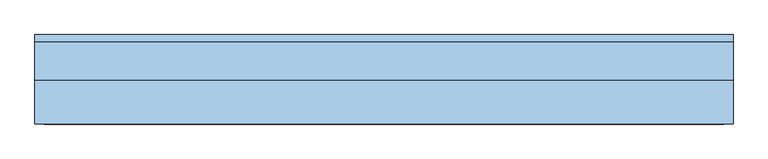
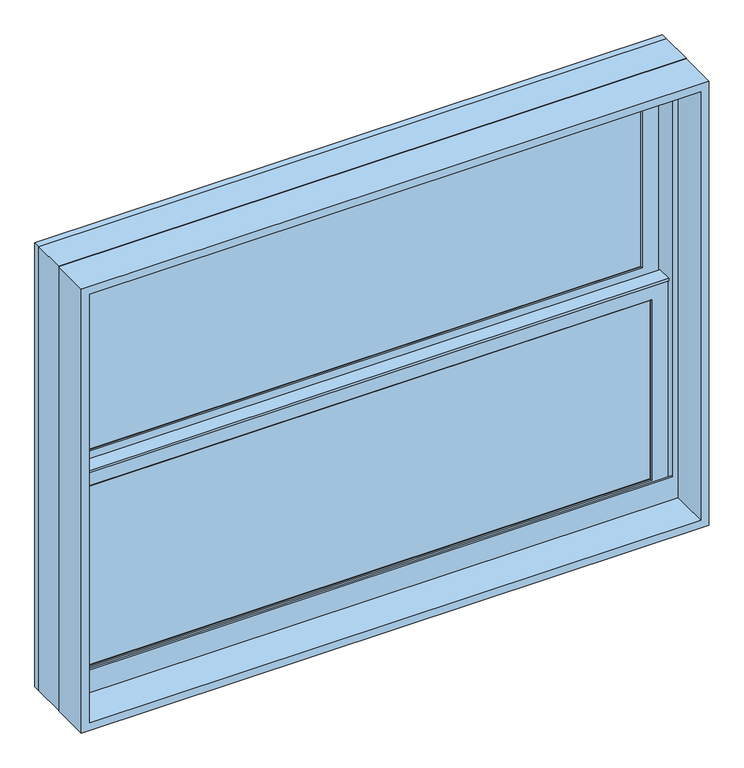
"""IFC4 building model written with IfcOpenShell, lengths in millimetres: window geometry, Window-Double_Hung-Marvin-Essential : ESDH4030."""

from ifc_helpers import new_model, si_unit, frame, origin, place, context, project, spatial, polyline, outline, extrude, faceted_brep, source, transform, mapped, element, save


def window_916ece20(model_context):
    return source(origin(), model_context, "Body", "SolidModel", [
        extrude(outline(polyline([(191.5583333, 20.6375), (191.5583333, 15.875), (172.5083333, 15.875), (172.5083333, 20.6375), (191.5583333, 20.6375)])), frame((0.0, 0.0, 1593.85), z_axis=(0.0, 0.0, 1.0), x_axis=(1.0, 0.0, 0.0)), (0.0, 0.0, 1.0), 374.65),
        extrude(outline(polyline([(-172.5083333, 20.6375), (-172.5083333, 15.875), (-191.5583333, 15.875), (-191.5583333, 20.6375), (-172.5083333, 20.6375)])), frame((0.0, 0.0, 1593.85), z_axis=(0.0, 0.0, 1.0), x_axis=(1.0, 0.0, 0.0)), (0.0, 0.0, 1.0), 374.65),
        extrude(outline(polyline([(546.1, 20.6375), (546.1, 15.875), (-546.1, 15.875), (-546.1, 20.6375), (546.1, 20.6375)])), frame((0.0, 0.0, 1771.65), z_axis=(0.0, 0.0, 1.0), x_axis=(1.0, 0.0, 0.0)), (0.0, 0.0, 1.0), 19.05),
        extrude(outline(polyline([(-191.5583333, 46.83125), (-191.5583333, 51.59375), (-172.5083333, 51.59375), (-172.5083333, 46.83125), (-191.5583333, 46.83125)])), frame((0.0, 0.0, 2006.6), z_axis=(0.0, 0.0, 1.0), x_axis=(1.0, 0.0, 0.0)), (0.0, 0.0, 1.0), 374.65),
        extrude(outline(polyline([(172.5083333, 46.83125), (172.5083333, 51.59375), (191.5583333, 51.59375), (191.5583333, 46.83125), (172.5083333, 46.83125)])), frame((0.0, 0.0, 2006.6), z_axis=(0.0, 0.0, 1.0), x_axis=(1.0, 0.0, 0.0)), (0.0, 0.0, 1.0), 374.65),
        extrude(outline(polyline([(-546.1, 46.83125), (-546.1, 51.59375), (546.1, 51.59375), (546.1, 46.83125), (-546.1, 46.83125)])), frame((0.0, 0.0, 2184.4), z_axis=(0.0, 0.0, 1.0), x_axis=(1.0, 0.0, 0.0)), (0.0, 0.0, 1.0), 19.05),
        extrude(outline(polyline([(191.5583333, 20.6375), (172.5083333, 20.6375), (172.5083333, 25.4), (191.5583333, 25.4), (191.5583333, 20.6375)])), frame((0.0, 0.0, 1593.85), z_axis=(0.0, 0.0, 1.0), x_axis=(1.0, 0.0, 0.0)), (0.0, 0.0, 1.0), 374.65),
        extrude(outline(polyline([(-172.5083333, 20.6375), (-191.5583333, 20.6375), (-191.5583333, 25.4), (-172.5083333, 25.4), (-172.5083333, 20.6375)])), frame((0.0, 0.0, 1593.85), z_axis=(0.0, 0.0, 1.0), x_axis=(1.0, 0.0, 0.0)), (0.0, 0.0, 1.0), 374.65),
        extrude(outline(polyline([(546.1, 20.6375), (-546.1, 20.6375), (-546.1, 25.4), (546.1, 25.4), (546.1, 20.6375)])), frame((0.0, 0.0, 1771.65), z_axis=(0.0, 0.0, 1.0), x_axis=(1.0, 0.0, 0.0)), (0.0, 0.0, 1.0), 19.05),
        extrude(outline(polyline([(-191.5583333, 56.35625), (-172.5083333, 56.35625), (-172.5083333, 51.59375), (-191.5583333, 51.59375), (-191.5583333, 56.35625)])), frame((0.0, 0.0, 2006.6), z_axis=(0.0, 0.0, 1.0), x_axis=(1.0, 0.0, 0.0)), (0.0, 0.0, 1.0), 374.65),
        extrude(outline(polyline([(172.5083333, 56.35625), (191.5583333, 56.35625), (191.5583333, 51.59375), (172.5083333, 51.59375), (172.5083333, 56.35625)])), frame((0.0, 0.0, 2006.6), z_axis=(0.0, 0.0, 1.0), x_axis=(1.0, 0.0, 0.0)), (0.0, 0.0, 1.0), 374.65),
        extrude(outline(polyline([(-546.1, 56.35625), (546.1, 56.35625), (546.1, 51.59375), (-546.1, 51.59375), (-546.1, 56.35625)])), frame((0.0, 0.0, 2184.4), z_axis=(0.0, 0.0, 1.0), x_axis=(1.0, 0.0, 0.0)), (0.0, 0.0, 1.0), 19.05),
        faceted_brep([(-573.0875, 5.6780605, 1998.5351748), (-573.0875, 5.6780605, 1993.9), (573.0875, 5.6780605, 1993.9), (573.0875, 5.6780605, 1998.5351748), (-573.0875, 34.8118605, 1998.5351748), (573.0875, 34.8118605, 1998.5351748), (573.0875, 34.8118605, 1993.9), (-573.0875, 34.8118605, 1993.9), (-573.0875, 30.1625, 1993.9), (-573.0875, 30.1625, 1566.8625), (-573.0875, 8.9241104, 1566.8625), (-573.0875, 8.9241104, 1993.9), (573.0875, 8.9241104, 1993.9), (573.0875, 30.1625, 1993.9), (573.0875, 8.9241104, 1566.8625), (573.0875, 30.1625, 1566.8625), (-557.2034752, 11.90625, 1979.6034752), (-557.2034752, 30.1625, 1979.6034752), (557.2034752, 30.1625, 1979.6034752), (557.2034752, 11.90625, 1979.6034752), (-540.54375, 10.4662439, 1962.94375), (-540.54375, 11.90625, 1962.94375), (540.54375, 11.90625, 1962.94375), (540.54375, 10.4662439, 1962.94375), (542.0858834, 8.9241104, 1964.4858834), (-542.0858834, 8.9241104, 1964.4858834), (557.2034752, 30.1625, 1582.7465248), (557.2034752, 11.90625, 1582.7465248), (540.54375, 11.90625, 1599.40625), (540.54375, 10.4662439, 1599.40625), (542.0858834, 8.9241104, 1597.8641166), (-557.2034752, 30.1625, 1582.7465248), (-557.2034752, 11.90625, 1582.7465248), (-540.54375, 11.90625, 1599.40625), (-540.54375, 10.4662439, 1599.40625), (-542.0858834, 8.9241104, 1597.8641166)], [[[0, 1, 2, 3]], [[4, 5, 6, 7]], [[1, 0, 4, 7, 8, 9, 10, 11]], [[2, 1, 11, 12]], [[7, 6, 13, 8]], [[3, 2, 12, 14, 15, 13, 6, 5]], [[0, 3, 5, 4]], [[16, 17, 18, 19]], [[20, 21, 22, 23]], [[20, 23, 24, 25]], [[19, 18, 26, 27]], [[23, 22, 28, 29]], [[24, 23, 29, 30]], [[27, 26, 31, 32]], [[29, 28, 33, 34]], [[30, 29, 34, 35]], [[15, 14, 10, 9]], [[15, 9, 8, 13], [18, 17, 31, 26]], [[17, 16, 32, 31]], [[16, 19, 27, 32], [22, 21, 33, 28]], [[21, 20, 34, 33]], [[20, 25, 35, 34]], [[10, 14, 12, 11], [25, 24, 30, 35]]]),
        extrude(outline(polyline([(38.5955581, 1979.6125), (33.5778968, 1979.6125), (33.5778968, 1981.2), (39.9405976, 1981.2), (39.9405976, 1979.6125), (61.515625, 1979.6125), (47.6307501, 1976.2975159), (38.5955581, 1976.2975159), (38.5955581, 1979.6125)])), frame((-573.0875, 0.0, 0.0), z_axis=(1.0, 0.0, 0.0), x_axis=(0.0, 1.0, 0.0)), (0.0, 0.0, 1.0), 1146.175),
        faceted_brep([(603.25, 0.0, 1536.7), (603.25, 0.0, 2438.4), (-603.25, 0.0, 2438.4), (-603.25, 0.0, 1536.7), (577.05625, 0.0, 1597.81875), (-577.05625, 0.0, 1597.81875), (-577.05625, 0.0, 2412.20625), (577.05625, 0.0, 2412.20625), (577.05625, 3.96875, 1536.7), (-577.05625, 3.96875, 1536.7), (-577.05625, 3.96875, 1597.81875), (577.05625, 3.96875, 1597.81875), (-603.25, 65.6828125, 1536.7), (-577.05625, 65.6828125, 1536.7), (577.05625, 65.6828125, 1536.7), (603.25, 65.6828125, 1536.7), (-603.25, 65.6828125, 2438.4), (603.25, 65.6828125, 2438.4), (577.05625, 65.6828125, 2412.20625), (-577.05625, 65.6828125, 2412.20625)], [[[0, 1, 2, 3], [4, 5, 6, 7]], [[8, 9, 10, 11]], [[5, 4, 11, 10]], [[0, 3, 12, 13, 9, 8, 14, 15]], [[13, 12, 16, 17, 15, 14, 18, 19]], [[13, 19, 6, 5, 10, 9]], [[7, 6, 19, 18]], [[18, 14, 8, 11, 4, 7]], [[1, 0, 15, 17]], [[2, 1, 17, 16]], [[3, 2, 16, 12]]]),
        faceted_brep([(577.05625, 30.1625, 1987.55), (575.46875, 30.1625, 1987.55), (575.46875, 30.1625, 1561.0544613), (577.05625, 30.1625, 1561.0544613), (-575.46875, 30.1625, 1987.55), (-577.05625, 30.1625, 1987.55), (-577.05625, 30.1625, 1561.0544613), (-575.46875, 30.1625, 1561.0544613), (575.46875, 63.5, 1987.55), (577.05625, 63.5, 1987.55), (577.05625, 63.5, 1554.5743077), (575.46875, 63.5, 1554.5743077), (-577.05625, 63.5, 1987.55), (-575.46875, 63.5, 1987.55), (-575.46875, 63.5, 1554.5743077), (-577.05625, 63.5, 1554.5743077), (588.3108932, 3.96875, 1566.1460105), (588.3108932, 3.96875, 1536.7), (588.3108932, 65.6828125, 1536.7), (588.3108932, 65.6828125, 1554.150012), (-588.3108932, 3.96875, 1536.7), (-588.3108932, 3.96875, 1566.1460105), (-588.3108932, 65.6828125, 1554.150012), (-588.3108932, 65.6828125, 1536.7), (588.3108932, 78.58125, 1551.6428097), (-588.3108932, 78.58125, 1551.6428097), (-586.2971252, 68.2348864, 1553.6539391), (-568.33135, 68.2348864, 1553.6539391), (-568.33135, 65.6828125, 1554.150012), (568.33135, 65.6828125, 1554.150012), (568.33135, 68.2348864, 1553.6539391), (586.2971252, 68.2348864, 1553.6539391), (-603.25, 65.6828125, 1536.7), (-603.25, 78.5948249, 1536.7), (603.25, 78.5948249, 1536.7), (603.25, 65.6828125, 1536.7), (-603.25, 78.58125, 2438.4), (603.25, 78.58125, 2438.4), (588.3108932, 78.58125, 2423.4608932), (-588.3108932, 78.58125, 2423.4608932), (-603.25, 65.6828125, 2438.4), (-586.2971252, 68.2348864, 2421.4471252), (586.2971252, 68.2348864, 2421.4471252), (568.33135, 68.2348864, 2403.48135), (-568.33135, 68.2348864, 2403.48135), (-568.33135, 65.6828125, 2403.48135), (568.33135, 65.6828125, 2403.48135), (603.25, 65.6828125, 2438.4)], [[[0, 1, 2, 3]], [[4, 5, 6, 7]], [[8, 9, 10, 11]], [[12, 13, 14, 15]], [[1, 8, 11, 2]], [[9, 0, 3, 10]], [[1, 0, 9, 8]], [[5, 4, 13, 12]], [[5, 12, 15, 6]], [[13, 4, 7, 14]], [[16, 17, 18, 19]], [[20, 21, 22, 23]], [[24, 25, 26, 27, 28, 22, 21, 16, 19, 29, 30, 31], [3, 2, 11, 10], [7, 6, 15, 14]], [[17, 16, 21, 20]], [[17, 20, 23, 32, 33, 34, 35, 18]], [[34, 33, 36, 37], [25, 24, 38, 39]], [[33, 32, 40, 36]], [[39, 41, 26, 25]], [[41, 42, 31, 30, 43, 44, 27, 26]], [[44, 45, 28, 27]], [[40, 32, 23, 22, 28, 45, 46, 29, 19, 18, 35, 47]], [[36, 40, 47, 37]], [[39, 38, 42, 41]], [[44, 43, 46, 45]], [[34, 37, 47, 35]], [[42, 38, 24, 31]], [[46, 43, 30, 29]]]),
        extrude(outline(polyline([(553.24375, 11.90625), (-553.24375, 11.90625), (-553.24375, 15.08125), (553.24375, 15.08125), (553.24375, 11.90625)])), frame((0.0, 0.0, 1586.70625), z_axis=(0.0, 0.0, 1.0), x_axis=(1.0, 0.0, 0.0)), (0.0, 0.0, 1.0), 388.9375),
        extrude(outline(polyline([(553.24375, 42.8625), (-553.24375, 42.8625), (-553.24375, 46.0375), (553.24375, 46.0375), (553.24375, 42.8625)])), frame((0.0, 0.0, 1999.45625), z_axis=(0.0, 0.0, 1.0), x_axis=(1.0, 0.0, 0.0)), (0.0, 0.0, 1.0), 388.9375),
        faceted_brep([(-540.54375, 31.194477, 1962.94375), (-542.0858834, 32.7366104, 1964.4858834), (542.0858834, 32.7366104, 1964.4858834), (540.54375, 31.194477, 1962.94375), (-540.54375, 30.1625, 1962.94375), (540.54375, 30.1625, 1962.94375), (-573.0875, 32.7366104, 1995.4875), (-573.0875, 30.1625, 1995.4875), (573.0875, 30.1625, 1995.4875), (573.0875, 32.7366104, 1995.4875), (542.0858834, 32.7366104, 1597.8641166), (540.54375, 31.194477, 1599.40625), (540.54375, 30.1625, 1599.40625), (573.0875, 30.1625, 1566.8625), (573.0875, 32.7366104, 1566.8625), (-542.0858834, 32.7366104, 1597.8641166), (-540.54375, 31.194477, 1599.40625), (-540.54375, 30.1625, 1599.40625), (-573.0875, 30.1625, 1566.8625), (-573.0875, 32.7366104, 1566.8625)], [[[0, 1, 2, 3]], [[4, 0, 3, 5]], [[6, 7, 8, 9]], [[3, 2, 10, 11]], [[5, 3, 11, 12]], [[9, 8, 13, 14]], [[11, 10, 15, 16]], [[12, 11, 16, 17]], [[14, 13, 18, 19]], [[9, 14, 19, 6], [1, 15, 10, 2]], [[16, 15, 1, 0]], [[17, 16, 0, 4]], [[7, 18, 13, 8], [5, 12, 17, 4]], [[19, 18, 7, 6]]]),
        faceted_brep([(-557.2034752, 42.8625, 2392.3534752), (-557.2034752, 61.11875, 2392.3534752), (557.2034752, 61.11875, 2392.3534752), (557.2034752, 42.8625, 2392.3534752), (-540.54375, 41.4224939, 2375.69375), (-540.54375, 42.8625, 2375.69375), (540.54375, 42.8625, 2375.69375), (540.54375, 41.4224939, 2375.69375), (-542.0858834, 39.8803604, 2377.2358834), (542.0858834, 39.8803604, 2377.2358834), (-573.0875, 61.11875, 2408.2375), (-573.0875, 39.8803604, 2408.2375), (573.0875, 39.8803604, 2408.2375), (573.0875, 61.11875, 2408.2375), (557.2034752, 61.11875, 1995.4965248), (557.2034752, 42.8625, 1995.4965248), (540.54375, 42.8625, 2012.15625), (540.54375, 41.4224939, 2012.15625), (542.0858834, 39.8803604, 2010.6141166), (573.0875, 39.8803604, 1979.6125), (573.0875, 61.11875, 1979.6125), (-557.2034752, 61.11875, 1995.4965248), (-557.2034752, 42.8625, 1995.4965248), (-540.54375, 42.8625, 2012.15625), (-540.54375, 41.4224939, 2012.15625), (-542.0858834, 39.8803604, 2010.6141166), (-573.0875, 39.8803604, 1979.6125), (-573.0875, 61.11875, 1979.6125)], [[[0, 1, 2, 3]], [[4, 5, 6, 7]], [[8, 4, 7, 9]], [[10, 11, 12, 13]], [[3, 2, 14, 15]], [[7, 6, 16, 17]], [[9, 7, 17, 18]], [[13, 12, 19, 20]], [[15, 14, 21, 22]], [[17, 16, 23, 24]], [[18, 17, 24, 25]], [[20, 19, 26, 27]], [[13, 20, 27, 10], [1, 21, 14, 2]], [[22, 21, 1, 0]], [[3, 15, 22, 0], [5, 23, 16, 6]], [[24, 23, 5, 4]], [[25, 24, 4, 8]], [[11, 26, 19, 12], [9, 18, 25, 8]], [[27, 26, 11, 10]]]),
        faceted_brep([(-573.0875, 61.11875, 1979.6125), (-573.0875, 63.6928604, 1979.6125), (573.0875, 63.6928604, 1979.6125), (573.0875, 61.11875, 1979.6125), (-540.54375, 62.150727, 2012.15625), (-540.54375, 61.11875, 2012.15625), (540.54375, 61.11875, 2012.15625), (540.54375, 62.150727, 2012.15625), (-542.0858834, 63.6928604, 2010.6141166), (542.0858834, 63.6928604, 2010.6141166), (573.0875, 63.6928604, 2408.2375), (573.0875, 61.11875, 2408.2375), (540.54375, 61.11875, 2375.69375), (540.54375, 62.150727, 2375.69375), (542.0858834, 63.6928604, 2377.2358834), (-573.0875, 63.6928604, 2408.2375), (-573.0875, 61.11875, 2408.2375), (-540.54375, 61.11875, 2375.69375), (-540.54375, 62.150727, 2375.69375), (-542.0858834, 63.6928604, 2377.2358834)], [[[0, 1, 2, 3]], [[4, 5, 6, 7]], [[8, 4, 7, 9]], [[3, 2, 10, 11]], [[7, 6, 12, 13]], [[9, 7, 13, 14]], [[11, 10, 15, 16]], [[13, 12, 17, 18]], [[14, 13, 18, 19]], [[16, 15, 1, 0]], [[3, 11, 16, 0], [5, 17, 12, 6]], [[18, 17, 5, 4]], [[19, 18, 4, 8]], [[1, 15, 10, 2], [9, 14, 19, 8]]]),
        extrude(outline(polyline([(553.24375, 26.19375), (-553.24375, 26.19375), (-553.24375, 30.1625), (553.24375, 30.1625), (553.24375, 26.19375)])), frame((0.0, 0.0, 1586.70625), z_axis=(0.0, 0.0, 1.0), x_axis=(1.0, 0.0, 0.0)), (0.0, 0.0, 1.0), 388.9375),
        extrude(outline(polyline([(553.24375, 57.15), (-553.24375, 57.15), (-553.24375, 61.11875), (553.24375, 61.11875), (553.24375, 57.15)])), frame((0.0, 0.0, 1999.45625), z_axis=(0.0, 0.0, 1.0), x_axis=(1.0, 0.0, 0.0)), (0.0, 0.0, 1.0), 388.9375),
        extrude(outline(polyline([(2438.4, 603.25), (2438.4, -603.25), (1536.7, -603.25), (1536.7, 603.25), (2438.4, 603.25)]), holes=[polyline([(2422.525, 587.375), (1552.575, 587.375), (1552.575, -587.375), (2422.525, -587.375), (2422.525, 587.375)])]), frame((0.0, -76.2, 0.0), z_axis=(0.0, 1.0, 0.0), x_axis=(0.0, 0.0, 1.0)), (0.0, 0.0, 1.0), 75.40625),
    ])


if __name__ == "__main__":
    model = new_model("IFC4")
    model_context = context("Model", 3, world=origin())
    ifc_project = project(units=[si_unit("LENGTHUNIT", "METRE", prefix="MILLI")], contexts=[model_context])
    site = spatial("IfcSite", under=ifc_project)
    building = spatial("IfcBuilding", under=site)
    placement = place(None, origin())
    window_shape = window_916ece20(model_context)
    element("IfcWindow", 1, ObjectType="Window-Double_Hung-Marvin-Essential : ESDH4030", at=placement, inside=building, context=model_context, shape_type="MappedRepresentation", body=[
        mapped(window_shape, transform((0.0, 0.0, 0.0), x_axis=(1.0, 0.0, 0.0), y_axis=(0.0, 1.0, 0.0), z_axis=(0.0, 0.0, 1.0))),
    ])
    save(model, "model.ifc")

# Revit data of these elements
# Type "Window-Double_Hung-Marvin-Essential : ESDH4030"
#   Type Mark = "39"
#   Window Type = "Essential Double Hung"
#   Product data url = "https://bimobject.com/marvin-windows-and-doors/product/marvin-dhwau"
#   Product Guid = "c4a96547-874c-4385-91dc-a058adc19d98"
#   Frame = "All Ultrex"
#   Egress Window = "No"
#   URL = "www.marvin.com"
#   Model = "ESDH4030"
#   Manufacturer = "Marvin Windows and Doors"
#   Label Egress = ""
#   Glass Type = "IG Low E II with Argon"
#   Design Pressure = "DP50"
#   Description = "4836 DBHG"
#   Analytic Construction = "<None>"
#   Prairie Corner Width = 0' - 4"
#   Prairie Corner Height = 0' - 4"
#   Egress Width = 3' - 8 9/16"
#   Egress Height = 1' - 1 27/128"
#   Rough Width = 4' - 0"
#   Rough Height = 3' - 0"
#   Nominal Width = 4' - 0"
#   Nominal Height = 3' - 0"
#   Inset to Installation Flange [instance default] = 0' - 1"
#   Height = 2' - 11 1/2"
#   Egress Area = 4.08828 SF
#   Default Head Height = 8' - 0"
#   Width = 3' - 11 1/2"
#   Daylight Area = 8.46077 SF
#   DLO Width = 3' - 6 9/16"
#   DLO Height = 1' - 2 5/16"
#   Muntins Top Sash = yes
#   Lites Wide Top Sash = 3
#   Lites Wide Bottom Sash = 3
#   Lites High Top Sash = 2
#   Lites High Bottom Sash = 2
#   Lite Cut Prairie 9 = no
#   Lite Cut HV Grid = yes
#   Muntins Bottom Sash = yes
#   Label Visibility = no
#   Jamb Extension Visibility = yes
#   Edition number = 1
#   Interior Material = Ultrex-Marvin-Stonewhite
#   Glazing Material = Glass-Marvin-IG Low E II with Argon
#   Cladding Material = Ultrex-Marvin-Pebblegray
#   Wall Closure = (empty or 0)
#   Assembly Code = ""
# Element 1 (IfcWindow, "Window-Double_Hung-Marvin-Essential : ESDH4030")
#   Materials on its faces: "Ultrex-Marvin-Pebblegray", "Ultrex-Marvin-Stonewhite", "Glass-Marvin-IG Low E II with Argon"
# Materials
#   "Ultrex-Marvin-Stonewhite": class "Paint", colour RGB 250 251 245, transparency 0
#   "Glass-Marvin-IG Low E II with Argon": class "Glass", colour RGB 0 128 192, transparency 0.85
#   "Ultrex-Marvin-Pebblegray": class "Paint", colour RGB 189 185 173, transparency 0
